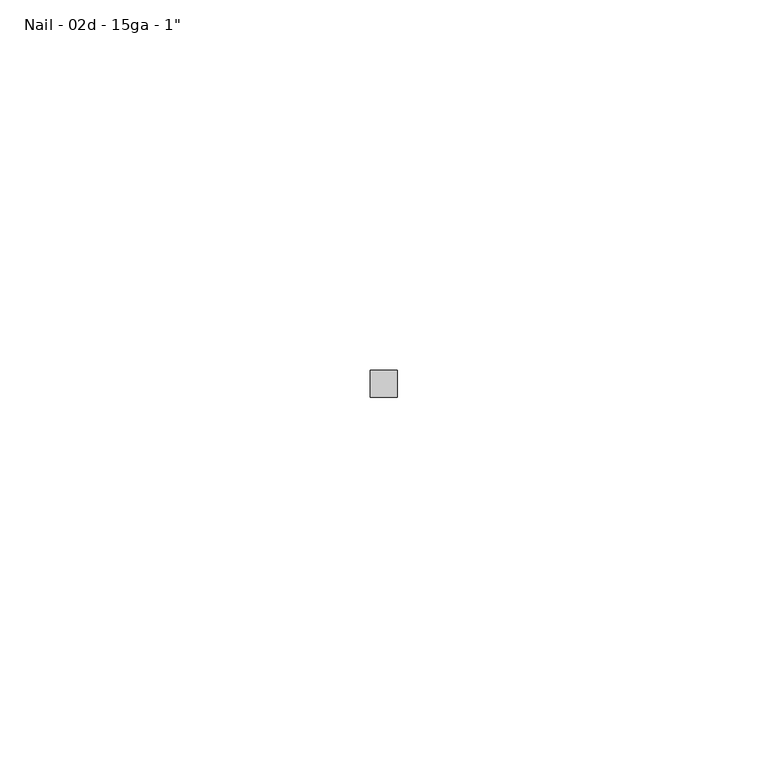
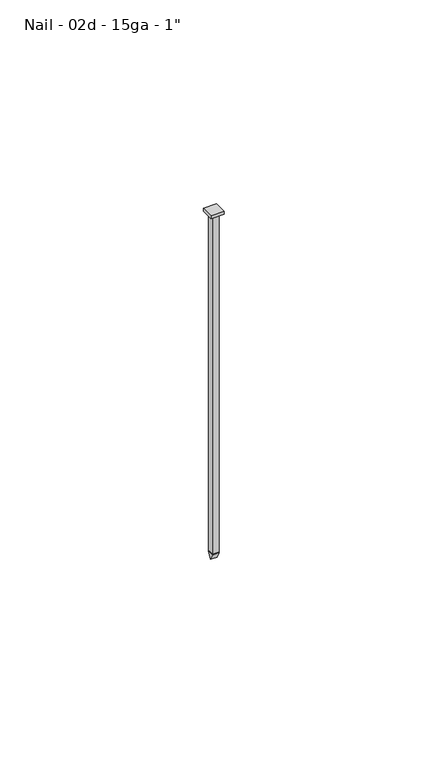
"""IFC4 building model written with IfcOpenShell, lengths in millimetres: fastener geometry."""

from ifc_helpers import new_model, si_unit, frame, origin, origin_with_axes, place, context, project, spatial, polyline, outline, extrude, source, transform, mapped, element, save


def fastener_da76262e(model_context):
    return source(origin(), model_context, "Body", "SweptSolid", [
        extrude(outline(polyline([(0.0, -103.4288), (-0.9144, -101.6), (0.9144, -101.6), (0.0, -103.4288)])), frame((-0.9144, 0.0, 0.0), z_axis=(1.0, 0.0, 0.0), x_axis=(0.0, 1.0, 0.0)), (0.0, 0.0, 1.0), 1.8288),
        extrude(outline(polyline([(-1.8288, -1.8288), (-1.8288, 1.8288), (1.8288, 1.8288), (1.8288, -1.8288), (-1.8288, -1.8288)])), origin_with_axes(), (0.0, 0.0, 1.0), 0.9144),
        extrude(outline(polyline([(-0.9144, 0.9144), (0.9144, 0.9144), (0.9144, -0.9144), (-0.9144, -0.9144), (-0.9144, 0.9144)])), frame((0.0, 0.0, -101.6), z_axis=(0.0, 0.0, 1.0), x_axis=(1.0, 0.0, 0.0)), (0.0, 0.0, 1.0), 101.6),
    ])


if __name__ == "__main__":
    model = new_model("IFC4")
    model_context = context("Model", 3, world=origin())
    ifc_project = project(units=[si_unit("LENGTHUNIT", "METRE", prefix="MILLI")], contexts=[model_context])
    site = spatial("IfcSite", under=ifc_project)
    building = spatial("IfcBuilding", under=site)
    placement = place(None, origin())
    fastener_shape = fastener_da76262e(model_context)
    element("IfcFastener", 1, ObjectType="060523 - W_P_C - Fastenings - Generic - SQUARE : Nail - 02d - 15ga - 1\"", at=placement, inside=building, context=model_context, shape_type="MappedRepresentation", body=[
        mapped(fastener_shape, transform((0.0, 0.0, 0.0), x_axis=(1.0, 0.0, 0.0), y_axis=(0.0, 1.0, 0.0), z_axis=(0.0, 0.0, 1.0))),
    ])
    save(model, "model.ifc")

# Revit data of these elements
# Type "060523 - W_P_C - Fastenings - Generic - SQUARE : Nail - 02d - 15ga - 1\""
#   Washer_Thickness = 0' - 0.00333"
#   Washer Radius = 0' - 0.046"
#   Washer Offset - Head = 0' - 0"
#   Washer Offset = 0' - 0"
#   Thickness_of_Substrate [instance default] = 0' - 1"
#   Side = 0' - 0 37/64"
#   Radius = 0' - 0.036"
#   Length [instance default] = 0' - 1"
#   Head Size = 0' - 1"
#   Head Radius = 0' - 0 1/2"
#   Head Height = 0' - 0.01"
#   Double Diameter = 0' - 0.144"
#   Diameter = 0' - 0.072"
#   Default Elevation = 4' - 0"
#   Washer_Nut_Visibility = no
#   Washer_Head_Visibility = no
#   Round_Head_Visibility = yes
#   Point Visibility = yes
#   Nut_Visibility = no
#   Hex_Head_Visiblilty = no
#   Washer Material = none
#   Bolt Material (Size) = AT SILL - FASTENER AT 24" O.C.
# Element 1 (IfcFastener, "060523 - W_P_C - Fastenings - Generic - SQUARE : Nail - 02d - 15ga - 1\"")
#   Length = 0' - 4"
# Materials
#   "AT SILL - FASTENER AT 24\" O.C.": class "Generic", colour RGB 120 120 120, transparency 0, Cost = 0
